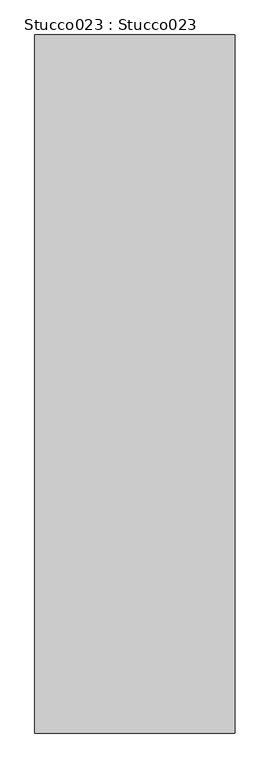
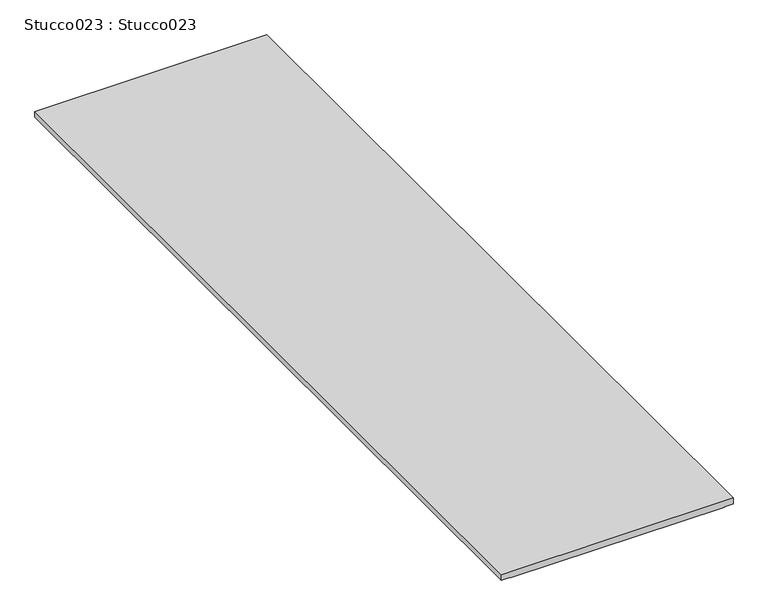
"""IFC4 building model written with IfcOpenShell, lengths in millimetres: proxy geometry, Stucco023 : Stucco023."""

from ifc_helpers import new_model, si_unit, frame, origin, place, context, project, spatial, polyline, outline, extrude, source, transform, mapped, element, save


def stucco023_stucco023_cbb9c5b5(model_context):
    return source(origin(), model_context, "Body", "SweptSolid", [
        extrude(outline(polyline([(39545.1675708, -4962.6175735), (39543.8875708, -4962.6175735), (39543.8875708, -4433.9671002), (39545.1675708, -4433.9671002), (39545.1675708, -4411.5339163), (39560.2460083, -4411.5339163), (39560.2460083, -4985.0507575), (39545.1675708, -4985.0507575), (39545.1675708, -4962.6175735)])), frame((0.0, -1052.8906574, 0.0), z_axis=(0.0, 1.0, 0.0), x_axis=(0.0, 0.0, 1.0)), (0.0, 0.0, 1.0), 2000.0),
    ])


if __name__ == "__main__":
    model = new_model("IFC4")
    model_context = context("Model", 3, world=origin())
    ifc_project = project(units=[si_unit("LENGTHUNIT", "METRE", prefix="MILLI")], contexts=[model_context])
    site = spatial("IfcSite", under=ifc_project)
    building = spatial("IfcBuilding", under=site)
    placement = place(None, origin())
    stucco023_stucco023_shape = stucco023_stucco023_cbb9c5b5(model_context)
    element("IfcBuildingElementProxy", 1, Name="Stucco023 : Stucco023", ObjectType="Stucco023 : Stucco023", at=placement, inside=building, context=model_context, shape_type="MappedRepresentation", body=[
        mapped(stucco023_stucco023_shape, transform((0.0, 0.0, 0.0), x_axis=(1.0, 0.0, 0.0), y_axis=(0.0, 1.0, 0.0), z_axis=(0.0, 0.0, 1.0))),
    ])
    save(model, "model.ifc")

# Revit data of these elements
# Type "Stucco023 : Stucco023"
#   NameOverride = "Stucco023"
# Element 1 (IfcBuildingElementProxy, "Stucco023 : Stucco023")
#   Materials on its faces: "7/8\" SMOOTH TROWEL EXTERIOR STUCCO"
# Materials
#   "7/8\" SMOOTH TROWEL EXTERIOR STUCCO": class "Unassigned", colour RGB 255 255 255, transparency 0, Cost = 0
